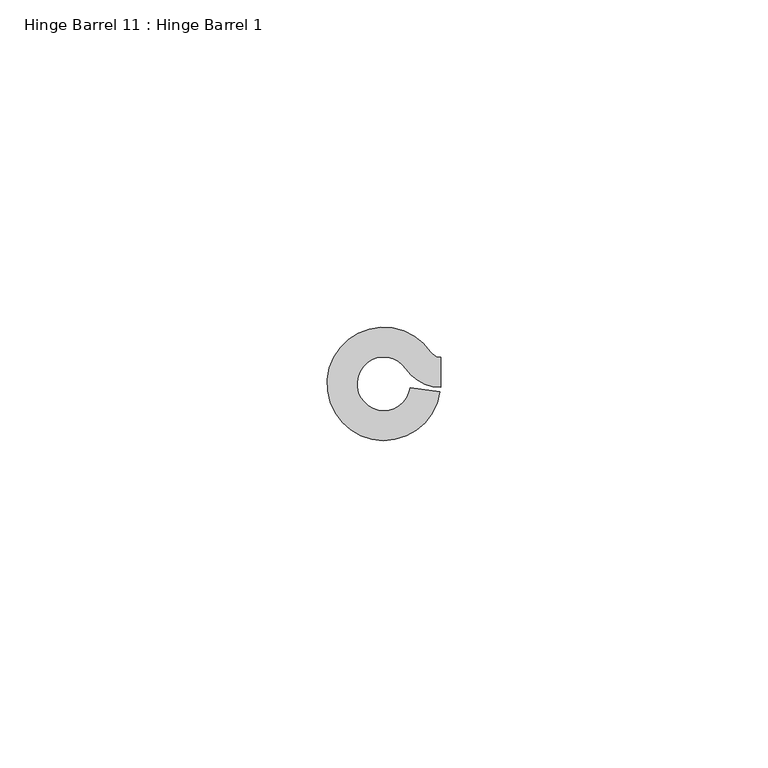
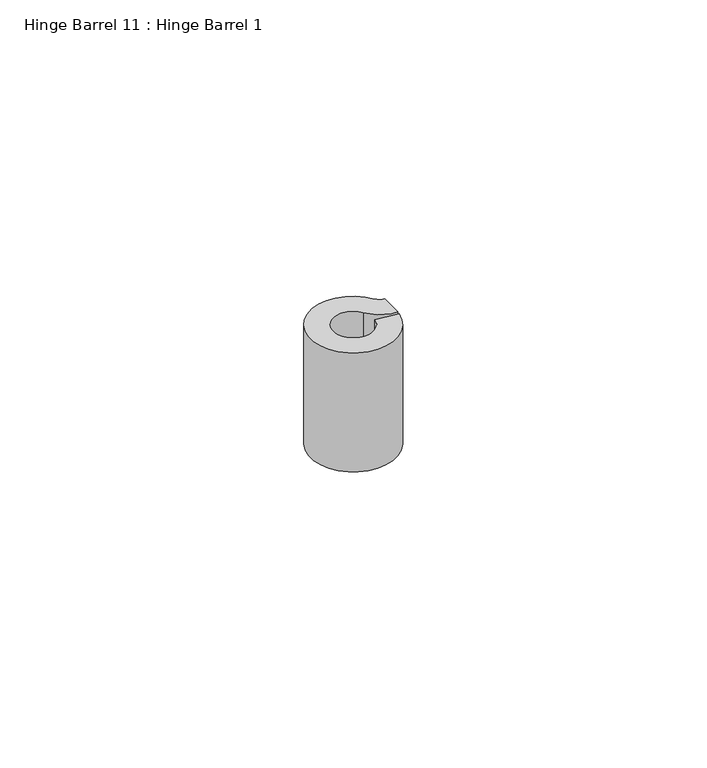
"""IFC4 building model written with IfcOpenShell, lengths in millimetres: proxy geometry, Hinge Barrel 11 : Hinge Barrel 1."""

from ifc_helpers import new_model, si_unit, point, frame, frame_2d, origin, place, context, project, spatial, polyline, circle_curve, trimmed, segment, composite_curve, outline, extrude, source, transform, mapped, element, save


def hinge_barrel_11_hinge_barrel_1_369d2be9(model_context):
    return source(origin(), model_context, "Body", "SweptSolid", [
        extrude(outline(composite_curve([segment(trimmed(circle_curve(frame_2d((587319.1320739, -531776.6049841)), 4.0894), [point((587322.5194669, -531774.3139665))], [point((587323.1821338, -531777.1708529))], True, "CARTESIAN"), True, "CONTINUOUS"), segment(polyline([(587323.1821338, -531777.1708529), (587327.7022899, -531777.8024028)]), True, "CONTINUOUS"), segment(trimmed(circle_curve(frame_2d((587319.1320739, -531776.6049841)), 8.6534625), [point((587327.7022899, -531777.8024028))], [point((587326.3000393, -531771.7570273))], False, "CARTESIAN"), True, "CONTINUOUS"), segment(trimmed(circle_curve(frame_2d((587327.8245257, -531770.7259615)), 1.8404226), [point((587326.3000393, -531771.7570273))], [point((587327.8245257, -531772.5663841))], True, "CARTESIAN"), True, "CONTINUOUS"), segment(polyline([(587327.8245257, -531772.5663841), (587327.8245257, -531777.1304466)]), True, "CONTINUOUS"), segment(trimmed(circle_curve(frame_2d((587327.8245257, -531770.7259615)), 6.4044851), [point((587327.8245257, -531777.1304466))], [point((587322.5194669, -531774.3139665))], False, "CARTESIAN"), True, "CONTINUOUS")], self_intersect=False)), frame((0.0, 0.0, 1962.15), z_axis=(0.0, 0.0, 1.0), x_axis=(1.0, 0.0, 0.0)), (0.0, 0.0, 1.0), 25.4),
    ])


if __name__ == "__main__":
    model = new_model("IFC4")
    model_context = context("Model", 3, world=origin())
    ifc_project = project(units=[si_unit("LENGTHUNIT", "METRE", prefix="MILLI")], contexts=[model_context])
    site = spatial("IfcSite", under=ifc_project)
    building = spatial("IfcBuilding", under=site)
    placement = place(None, origin())
    hinge_barrel_11_hinge_barrel_1_shape = hinge_barrel_11_hinge_barrel_1_369d2be9(model_context)
    element("IfcBuildingElementProxy", 1, Name="Hinge Barrel 11 : Hinge Barrel 1", ObjectType="Hinge Barrel 11 : Hinge Barrel 1", at=placement, inside=building, context=model_context, shape_type="MappedRepresentation", body=[
        mapped(hinge_barrel_11_hinge_barrel_1_shape, transform((0.0, 0.0, 0.0), x_axis=(1.0, 0.0, 0.0), y_axis=(0.0, 1.0, 0.0), z_axis=(0.0, 0.0, 1.0))),
    ])
    save(model, "model.ifc")

# Revit data of these elements
# Element 1 (IfcBuildingElementProxy, "Hinge Barrel 11 : Hinge Barrel 1")
#   Materials on its faces: "6\"X6\" WELD-ON STL BUTT HINGE"
# Materials
#   "6\"X6\" WELD-ON STL BUTT HINGE": class "Metal", colour RGB 189 187 185, transparency 0, Description = "Carbon steel", Cost = 0
